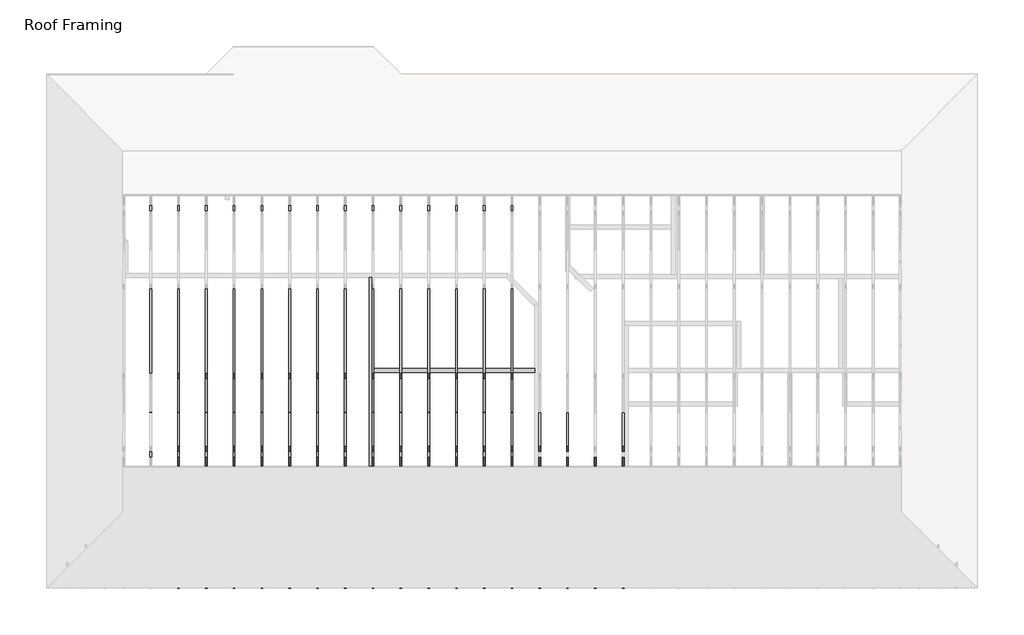
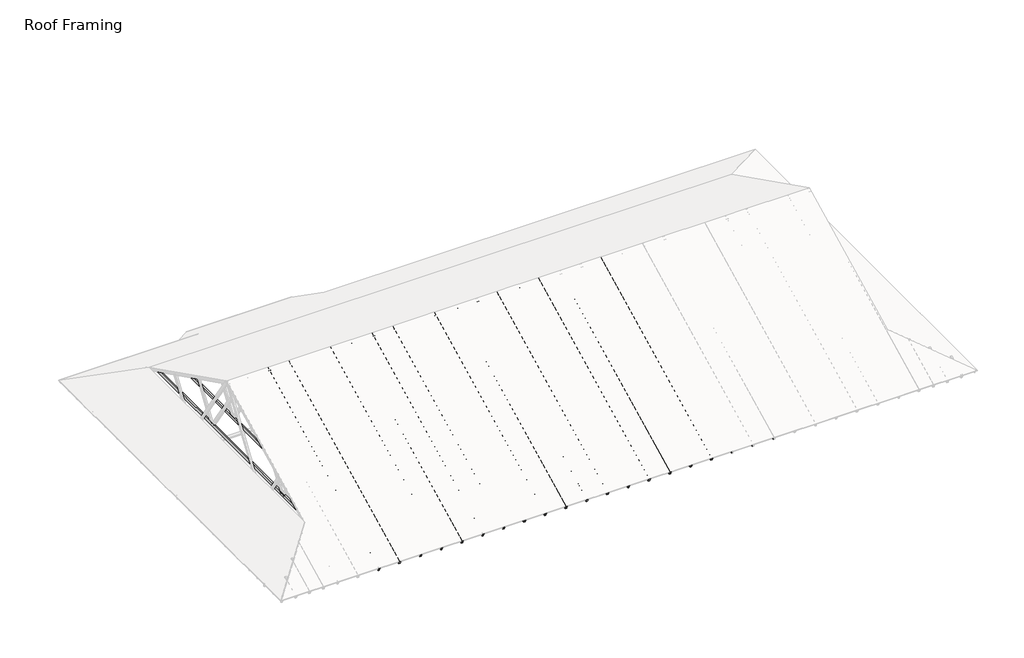
# One storey, part 2 of 7: 49 beams, 29 members.
"""IFC4 building model written with IfcOpenShell, lengths in millimetres."""

import ifcopenshell
import ifcopenshell.guid

model = None  # the IFC model being written
_history = None  # IfcOwnerHistory: only IFC2X3 demands one
_inside = {}  # id of a spatial element -> (the spatial element, [elements in it])
_under = {}  # id of a project, library or spatial element -> (it, [spatial elements below it])
_declared = {}  # id of a project -> (the project, [libraries it declares])
_typed = {}  # id of a type object -> (the type object, [elements of that type])
_made_of = {}  # id of a material, layer set ... -> (it, [elements and type objects made of it])


def new_model(schema):
    """Start an empty IFC model of exactly this schema.

    Asked for "IFC4X3", IfcOpenShell would pick the latest addendum, in which some entities
    have other attributes; the version numbers below select the first issue.
    IFC2X3 requires an IfcOwnerHistory on every rooted entity: one is made here for all.
    """
    global model, _history
    if schema == "IFC4X3":
        model = ifcopenshell.file(schema_version=(4, 3, 0, 0))
    else:
        model = ifcopenshell.file(schema=schema)
    _inside.clear()
    _under.clear()
    _declared.clear()
    _typed.clear()
    _made_of.clear()
    _history = None
    if model.schema == "IFC2X3":
        org = make("IfcOrganization", Name="unknown")
        user = make(
            "IfcPersonAndOrganization",
            ThePerson=make("IfcPerson", FamilyName="unknown"),
            TheOrganization=org,
        )
        app = make(
            "IfcApplication",
            ApplicationDeveloper=org,
            Version="unknown",
            ApplicationFullName="unknown",
            ApplicationIdentifier="unknown",
        )
        _history = make(
            "IfcOwnerHistory",
            OwningUser=user,
            OwningApplication=app,
            ChangeAction="ADDED",
            CreationDate=0,
        )
    return model


def make(cls, **values):
    """One entity of the class cls with the attributes given. An attribute that is None is left unset."""
    return model.create_entity(
        cls, **{name: value for name, value in values.items() if value is not None}
    )


def rooted(cls, **values):
    """An entity with a GlobalId (a new one), such as an element, a storey or a relation."""
    return make(cls, GlobalId=ifcopenshell.guid.new(), OwnerHistory=_history, **values)


def si_unit(unit_type, name, prefix=None):
    """IfcSIUnit, for example si_unit("LENGTHUNIT", "METRE", prefix="MILLI")."""
    return make("IfcSIUnit", UnitType=unit_type, Prefix=prefix, Name=name)


def assignment(units):
    """IfcUnitAssignment: the units of a project."""
    return None if units is None else make("IfcUnitAssignment", Units=units)


def point(xyz):
    """IfcCartesianPoint."""
    return None if xyz is None else make("IfcCartesianPoint", Coordinates=xyz)


def direction(xyz):
    """IfcDirection."""
    return None if xyz is None else make("IfcDirection", DirectionRatios=xyz)


def frame(location, z_axis=None, x_axis=None):
    """IfcAxis2Placement3D, a coordinate frame: its origin and axes. An axis left out is left unset."""
    return make(
        "IfcAxis2Placement3D",
        Location=point(location),
        Axis=direction(z_axis),
        RefDirection=direction(x_axis),
    )


def origin():
    """The frame at (0, 0, 0) with its axes left unset."""
    return frame((0.0, 0.0, 0.0))


def place(relative_to, where):
    """IfcLocalPlacement: puts the frame where relative to a parent placement (None: the world)."""
    return make(
        "IfcLocalPlacement", PlacementRelTo=relative_to, RelativePlacement=where
    )


def context(
    kind, dimensions, precision=None, world=None, true_north=None, identifier=None
):
    """IfcGeometricRepresentationContext, for example the 3D "Model" context."""
    return make(
        "IfcGeometricRepresentationContext",
        ContextIdentifier=identifier,
        ContextType=kind,
        CoordinateSpaceDimension=dimensions,
        Precision=precision,
        WorldCoordinateSystem=world,
        TrueNorth=true_north,
    )


def project(units=None, contexts=None):
    """IfcProject with its units and contexts."""
    return rooted(
        "IfcProject",
        Name="project",
        RepresentationContexts=contexts,
        UnitsInContext=assignment(units),
    )


def spatial(cls, under=None, at=None, **own):
    """A site, building, storey or space (cls), placed at a placement, below another one or the project."""
    s = rooted(cls, ObjectPlacement=at, **own)
    if under is not None:
        _under.setdefault(under.id(), (under, []))[1].append(s)
    return s


def polyline(points):
    """IfcPolyline through the points."""
    return make("IfcPolyline", Points=[point(p) for p in points])


def outline(outer, holes=None, kind="AREA"):
    """IfcArbitraryClosedProfileDef: a profile drawn as a closed curve; with holes, ...WithVoids."""
    if holes is None:
        return make("IfcArbitraryClosedProfileDef", ProfileType=kind, OuterCurve=outer)
    return make(
        "IfcArbitraryProfileDefWithVoids",
        ProfileType=kind,
        OuterCurve=outer,
        InnerCurves=holes,
    )


def extrude(swept, where, along, depth):
    """IfcExtrudedAreaSolid: the profile swept, set in the frame where, extruded along a direction by depth."""
    return make(
        "IfcExtrudedAreaSolid",
        SweptArea=swept,
        Position=where,
        ExtrudedDirection=direction(along),
        Depth=depth,
    )


def shape(context_of_items, identifier, shape_type, items):
    """IfcShapeRepresentation: the items that make up one representation, for example the "Body"."""
    return make(
        "IfcShapeRepresentation",
        ContextOfItems=context_of_items,
        RepresentationIdentifier=identifier,
        RepresentationType=shape_type,
        Items=items,
    )


def source(mapping_origin, context_of_items, identifier, shape_type, items):
    """IfcRepresentationMap: a shape defined once, which mapped items show again and again."""
    return make(
        "IfcRepresentationMap",
        MappingOrigin=mapping_origin,
        MappedRepresentation=shape(context_of_items, identifier, shape_type, items),
    )


def transform(
    local_origin,
    x_axis=None,
    y_axis=None,
    z_axis=None,
    scale=None,
    scale2=None,
    scale3=None,
    uniform=True,
):
    """IfcCartesianTransformationOperator3D, or its non-uniform kind. x_axis, y_axis, z_axis: its Axis1, 2, 3."""
    if uniform:
        return make(
            "IfcCartesianTransformationOperator3D",
            Axis1=direction(x_axis),
            Axis2=direction(y_axis),
            LocalOrigin=point(local_origin),
            Scale=scale,
            Axis3=direction(z_axis),
        )
    return make(
        "IfcCartesianTransformationOperator3DnonUniform",
        Axis1=direction(x_axis),
        Axis2=direction(y_axis),
        LocalOrigin=point(local_origin),
        Scale=scale,
        Axis3=direction(z_axis),
        Scale2=scale2,
        Scale3=scale3,
    )


def mapped(mapping_source, mapping_target):
    """IfcMappedItem: shows the shape of a source again, moved by a transform."""
    return make(
        "IfcMappedItem", MappingSource=mapping_source, MappingTarget=mapping_target
    )


def made_of(thing, what):
    """Note that an element or type object is made of a material, layer set ...; save() writes the relation."""
    if what is not None:
        _made_of.setdefault(what.id(), (what, []))[1].append(thing)
    return thing


def element(
    cls,
    number,
    at=None,
    inside=None,
    cuts=None,
    type_object=None,
    material=None,
    context=None,
    identifier="Body",
    shape_type=None,
    held_by="IfcProductDefinitionShape",
    body=None,
    shapes=None,
    **own,
):
    """One element of the class cls, such as IfcWall. Its Tag is "e" and its number.

    at: its placement. inside: the storey or other place that contains it. cuts: it is an
    opening in that element (IfcRelVoidsElement). A single representation is given by context,
    identifier, shape_type and body (its items); several are given by shapes. held_by: the class
    of the entity that holds the representations. save() writes the other relations.
    """
    e = rooted(cls, Tag="e%d" % number, ObjectPlacement=at, **own)
    if body is not None:
        shapes = [shape(context, identifier, shape_type, body)]
    if shapes is not None:
        e.Representation = make(held_by, Representations=shapes)
    if inside is not None:
        _inside.setdefault(inside.id(), (inside, []))[1].append(e)
    if cuts is not None:
        rooted(
            "IfcRelVoidsElement", RelatingBuildingElement=cuts, RelatedOpeningElement=e
        )
    if type_object is not None:
        _typed.setdefault(type_object.id(), (type_object, []))[1].append(e)
    return made_of(e, material)


def aggregate(whole, parts):
    """IfcRelAggregates: a whole, such as a stair, and the parts it consists of."""
    return rooted("IfcRelAggregates", RelatingObject=whole, RelatedObjects=parts)


def save(model, path):
    """Write the relations noted so far, then the file.

    IfcRelAggregates (storeys below a building ...), IfcRelContainedInSpatialStructure (elements
    in a storey), IfcRelDefinesByType, IfcRelAssociatesMaterial and IfcRelDeclares: one each for
    every whole, place, type object, material and project.
    """
    for whole, parts in _under.values():
        aggregate(whole, parts)
    for where, things in _inside.values():
        rooted(
            "IfcRelContainedInSpatialStructure",
            RelatedElements=things,
            RelatingStructure=where,
        )
    for kind, things in _typed.values():
        rooted("IfcRelDefinesByType", RelatedObjects=things, RelatingType=kind)
    for what, things in _made_of.values():
        rooted("IfcRelAssociatesMaterial", RelatedObjects=things, RelatingMaterial=what)
    for by, libraries in _declared.values():
        rooted("IfcRelDeclares", RelatingContext=by, RelatedDefinitions=libraries)
    model.write(path)


def dimension_lumber_f19b9f83(model_context):
    return source(origin(), model_context, "Body", "SweptSolid", [
        extrude(outline(polyline([(13763.625, -19.05), (-5743.575, -19.05), (-5743.575, 19.05), (13763.625, 19.05), (13763.625, -19.05)])), frame((0.0, 0.0, -44.45), z_axis=(0.0, 0.0, 1.0), x_axis=(1.0, 0.0, 0.0)), (0.0, 0.0, 1.0), 88.9),
    ])


def dimension_lumber_59ffca9e(model_context):
    return source(origin(), model_context, "Body", "SweptSolid", [
        extrude(outline(polyline([(1028.7, 44.45), (1028.7, -44.45), (-1028.7, -44.45), (-1028.7, 44.45), (1028.7, 44.45)])), frame((0.0, 0.0, -19.05), z_axis=(0.0, 0.0, 1.0), x_axis=(1.0, 0.0, 0.0)), (0.0, 0.0, 1.0), 38.1),
    ])


def dimension_lumber_a9f99430(model_context):
    return source(origin(), model_context, "Body", "SweptSolid", [
        extrude(outline(polyline([(1762.125, 44.45), (1762.125, -44.45), (-1778.0, -44.45), (-1778.0, 44.45), (1762.125, 44.45)])), frame((0.0, 0.0, -19.05), z_axis=(0.0, 0.0, 1.0), x_axis=(1.0, 0.0, 0.0)), (0.0, 0.0, 1.0), 38.1),
    ])


def dimension_lumber_f5869125(model_context):
    return source(origin(), model_context, "Body", "SweptSolid", [
        extrude(outline(polyline([(3033.7125, 44.45), (3033.7125, -44.45), (-3116.2625, -44.45), (-3116.2625, 44.45), (3033.7125, 44.45)])), frame((0.0, 0.0, -19.05), z_axis=(0.0, 0.0, 1.0), x_axis=(1.0, 0.0, 0.0)), (0.0, 0.0, 1.0), 38.1),
    ])


model = new_model("IFC4")

# Units and contexts
model_context = context("Model", 3, world=origin())
ifc_project = project(units=[si_unit("LENGTHUNIT", "METRE", prefix="MILLI")], contexts=[model_context])

# Site, building, storey
site = spatial("IfcSite", under=ifc_project)
building = spatial("IfcBuilding", under=site)
storey = spatial("IfcBuildingStorey", under=building, Name="Roof Framing", Elevation=2768.6)

# Beams
placement = place(None, origin())
dimension_lumber_shape = dimension_lumber_f19b9f83(model_context)
element("IfcBeam", 1, ObjectType="Dimension Lumber : Roof Lumbers", at=placement, inside=storey, context=model_context, shape_type="MappedRepresentation", body=[
    mapped(dimension_lumber_shape, transform((7511.6097749, -5882.9040947, 2609.05625), x_axis=(-1.0, 0.0, 0.0), y_axis=(0.0, -1.0, 0.0), z_axis=(0.0, 0.0, 1.0))),
])
dimension_lumber_2_shape = dimension_lumber_59ffca9e(model_context)
element("IfcBeam", 2, ObjectType="Dimension Lumber : Top Supporting Lumbers", at=placement, inside=storey, context=model_context, shape_type="MappedRepresentation", body=[
    mapped(dimension_lumber_2_shape, transform((5025.5847749, -4282.7040947, 2749.55), x_axis=(1.0, 0.0, 0.0), y_axis=(0.0, 1.0, 0.0), z_axis=(0.0, 0.0, 1.0))),
])
element("IfcBeam", 3, ObjectType="Dimension Lumber : Top Supporting Lumbers", at=placement, inside=storey, context=model_context, shape_type="MappedRepresentation", body=[
    mapped(dimension_lumber_2_shape, transform((5025.5847749, -4282.7040947, 2711.45), x_axis=(1.0, 0.0, 0.0), y_axis=(0.0, 1.0, 0.0), z_axis=(0.0, 0.0, 1.0))),
])
dimension_lumber_3_shape = dimension_lumber_a9f99430(model_context)
element("IfcBeam", 4, ObjectType="Dimension Lumber : Top Supporting Lumbers", at=placement, inside=storey, context=model_context, shape_type="MappedRepresentation", body=[
    mapped(dimension_lumber_3_shape, transform((2234.7597749, -1545.8540947, 2711.45), x_axis=(1.0, 0.0, 0.0), y_axis=(0.0, 1.0, 0.0), z_axis=(0.0, 0.0, 1.0))),
])
dimension_lumber_4_shape = dimension_lumber_f5869125(model_context)
element("IfcBeam", 5, ObjectType="Dimension Lumber : Top Supporting Lumbers", at=placement, inside=storey, context=model_context, shape_type="MappedRepresentation", body=[
    mapped(dimension_lumber_4_shape, transform((412.3097749, -2544.3915947, 2711.45), x_axis=(0.0, 1.0, 0.0), y_axis=(-1.0, 0.0, 0.0), z_axis=(0.0, 0.0, 1.0))),
])
element("IfcBeam", 6, ObjectType="Dimension Lumber : 2x4 Blocking", at=placement, inside=storey, context=model_context, shape_type="SweptSolid", body=[
    extrude(outline(polyline([(7787.8347749, -6282.9540947), (7749.7347749, -6282.9540947), (7749.7347749, -5901.9540947), (7787.8347749, -5901.9540947), (7787.8347749, -6282.9540947)])), frame((0.0, 0.0, 2564.60625), z_axis=(0.0, 0.0, 1.0), x_axis=(1.0, 0.0, 0.0)), (0.0, 0.0, 1.0), 88.9),
    extrude(outline(polyline([(-6083.9649001, 2653.50625), (-5901.9540947, 2653.50625), (-5901.9540947, 2564.60625), (-6261.7649001, 2564.60625), (-6083.9649001, 2653.50625)])), frame((7749.7347749, 0.0, 0.0), z_axis=(1.0, 0.0, 0.0), x_axis=(0.0, 1.0, 0.0)), (0.0, 0.0, 1.0), 38.1),
])
element("IfcBeam", 7, ObjectType="Dimension Lumber : 2x4 Blocking", at=placement, inside=storey, context=model_context, shape_type="SweptSolid", body=[
    extrude(outline(polyline([(7178.2347749, -6282.9540947), (7140.1347749, -6282.9540947), (7140.1347749, -5901.9540947), (7178.2347749, -5901.9540947), (7178.2347749, -6282.9540947)])), frame((0.0, 0.0, 2564.60625), z_axis=(0.0, 0.0, 1.0), x_axis=(1.0, 0.0, 0.0)), (0.0, 0.0, 1.0), 88.9),
    extrude(outline(polyline([(-6083.9649001, 2653.50625), (-5901.9540947, 2653.50625), (-5901.9540947, 2564.60625), (-6261.7649001, 2564.60625), (-6083.9649001, 2653.50625)])), frame((7140.1347749, 0.0, 0.0), z_axis=(1.0, 0.0, 0.0), x_axis=(0.0, 1.0, 0.0)), (0.0, 0.0, 1.0), 38.1),
])
element("IfcBeam", 8, ObjectType="Dimension Lumber : 2x4 Blocking", at=placement, inside=storey, context=model_context, shape_type="SweptSolid", body=[
    extrude(outline(polyline([(6568.6347749, -6282.9540947), (6530.5347749, -6282.9540947), (6530.5347749, -5901.9540947), (6568.6347749, -5901.9540947), (6568.6347749, -6282.9540947)])), frame((0.0, 0.0, 2564.60625), z_axis=(0.0, 0.0, 1.0), x_axis=(1.0, 0.0, 0.0)), (0.0, 0.0, 1.0), 88.9),
    extrude(outline(polyline([(-6083.9649001, 2653.50625), (-5901.9540947, 2653.50625), (-5901.9540947, 2564.60625), (-6261.7649001, 2564.60625), (-6083.9649001, 2653.50625)])), frame((6530.5347749, 0.0, 0.0), z_axis=(1.0, 0.0, 0.0), x_axis=(0.0, 1.0, 0.0)), (0.0, 0.0, 1.0), 38.1),
])
element("IfcBeam", 9, ObjectType="Dimension Lumber : 2x4 Blocking", at=placement, inside=storey, context=model_context, shape_type="SweptSolid", body=[
    extrude(outline(polyline([(5959.0347749, -6282.9540947), (5920.9347749, -6282.9540947), (5920.9347749, -5901.9540947), (5959.0347749, -5901.9540947), (5959.0347749, -6282.9540947)])), frame((0.0, 0.0, 2564.60625), z_axis=(0.0, 0.0, 1.0), x_axis=(1.0, 0.0, 0.0)), (0.0, 0.0, 1.0), 88.9),
    extrude(outline(polyline([(-6083.9649001, 2653.50625), (-5901.9540947, 2653.50625), (-5901.9540947, 2564.60625), (-6261.7649001, 2564.60625), (-6083.9649001, 2653.50625)])), frame((5920.9347749, 0.0, 0.0), z_axis=(1.0, 0.0, 0.0), x_axis=(0.0, 1.0, 0.0)), (0.0, 0.0, 1.0), 38.1),
])
element("IfcBeam", 10, ObjectType="Dimension Lumber : 2x4 Blocking", at=placement, inside=storey, context=model_context, shape_type="SweptSolid", body=[
    extrude(outline(polyline([(5349.4347749, -6282.9540947), (5311.3347749, -6282.9540947), (5311.3347749, -5901.9540947), (5349.4347749, -5901.9540947), (5349.4347749, -6282.9540947)])), frame((0.0, 0.0, 2564.60625), z_axis=(0.0, 0.0, 1.0), x_axis=(1.0, 0.0, 0.0)), (0.0, 0.0, 1.0), 88.9),
    extrude(outline(polyline([(-6083.9649001, 2653.50625), (-5901.9540947, 2653.50625), (-5901.9540947, 2564.60625), (-6261.7649001, 2564.60625), (-6083.9649001, 2653.50625)])), frame((5311.3347749, 0.0, 0.0), z_axis=(1.0, 0.0, 0.0), x_axis=(0.0, 1.0, 0.0)), (0.0, 0.0, 1.0), 38.1),
])
element("IfcBeam", 11, ObjectType="Dimension Lumber : 2x4 Blocking", at=placement, inside=storey, context=model_context, shape_type="SweptSolid", body=[
    extrude(outline(polyline([(4739.8347749, -6282.9540947), (4701.7347749, -6282.9540947), (4701.7347749, -5901.9540947), (4739.8347749, -5901.9540947), (4739.8347749, -6282.9540947)])), frame((0.0, 0.0, 2564.60625), z_axis=(0.0, 0.0, 1.0), x_axis=(1.0, 0.0, 0.0)), (0.0, 0.0, 1.0), 88.9),
    extrude(outline(polyline([(-6083.9649001, 2653.50625), (-5901.9540947, 2653.50625), (-5901.9540947, 2564.60625), (-6261.7649001, 2564.60625), (-6083.9649001, 2653.50625)])), frame((4701.7347749, 0.0, 0.0), z_axis=(1.0, 0.0, 0.0), x_axis=(0.0, 1.0, 0.0)), (0.0, 0.0, 1.0), 38.1),
])
element("IfcBeam", 12, ObjectType="Dimension Lumber : 2x4 Blocking", at=placement, inside=storey, context=model_context, shape_type="SweptSolid", body=[
    extrude(outline(polyline([(4130.2347749, -6282.9540947), (4092.1347749, -6282.9540947), (4092.1347749, -5901.9540947), (4130.2347749, -5901.9540947), (4130.2347749, -6282.9540947)])), frame((0.0, 0.0, 2564.60625), z_axis=(0.0, 0.0, 1.0), x_axis=(1.0, 0.0, 0.0)), (0.0, 0.0, 1.0), 88.9),
    extrude(outline(polyline([(-6083.9649001, 2653.50625), (-5901.9540947, 2653.50625), (-5901.9540947, 2564.60625), (-6261.7649001, 2564.60625), (-6083.9649001, 2653.50625)])), frame((4092.1347749, 0.0, 0.0), z_axis=(1.0, 0.0, 0.0), x_axis=(0.0, 1.0, 0.0)), (0.0, 0.0, 1.0), 38.1),
])
element("IfcBeam", 13, ObjectType="Dimension Lumber : 2x4 Blocking", at=placement, inside=storey, context=model_context, shape_type="SweptSolid", body=[
    extrude(outline(polyline([(3520.6347749, -6282.9540947), (3482.5347749, -6282.9540947), (3482.5347749, -5901.9540947), (3520.6347749, -5901.9540947), (3520.6347749, -6282.9540947)])), frame((0.0, 0.0, 2564.60625), z_axis=(0.0, 0.0, 1.0), x_axis=(1.0, 0.0, 0.0)), (0.0, 0.0, 1.0), 88.9),
    extrude(outline(polyline([(-6083.9649001, 2653.50625), (-5901.9540947, 2653.50625), (-5901.9540947, 2564.60625), (-6261.7649001, 2564.60625), (-6083.9649001, 2653.50625)])), frame((3482.5347749, 0.0, 0.0), z_axis=(1.0, 0.0, 0.0), x_axis=(0.0, 1.0, 0.0)), (0.0, 0.0, 1.0), 38.1),
])
element("IfcBeam", 14, ObjectType="Dimension Lumber : 2x4 Blocking", at=placement, inside=storey, context=model_context, shape_type="SweptSolid", body=[
    extrude(outline(polyline([(2911.0347749, -6282.9540947), (2872.9347749, -6282.9540947), (2872.9347749, -5901.9540947), (2911.0347749, -5901.9540947), (2911.0347749, -6282.9540947)])), frame((0.0, 0.0, 2564.60625), z_axis=(0.0, 0.0, 1.0), x_axis=(1.0, 0.0, 0.0)), (0.0, 0.0, 1.0), 88.9),
    extrude(outline(polyline([(-6083.9649001, 2653.50625), (-5901.9540947, 2653.50625), (-5901.9540947, 2564.60625), (-6261.7649001, 2564.60625), (-6083.9649001, 2653.50625)])), frame((2872.9347749, 0.0, 0.0), z_axis=(1.0, 0.0, 0.0), x_axis=(0.0, 1.0, 0.0)), (0.0, 0.0, 1.0), 38.1),
])
element("IfcBeam", 15, ObjectType="Dimension Lumber : 2x4 Blocking", at=placement, inside=storey, context=model_context, shape_type="SweptSolid", body=[
    extrude(outline(polyline([(2263.3347749, -5901.9540947), (2301.4347749, -5901.9540947), (2301.4347749, -6282.9540947), (2263.3347749, -6282.9540947), (2263.3347749, -5901.9540947)])), frame((0.0, 0.0, 2564.60625), z_axis=(0.0, 0.0, 1.0), x_axis=(1.0, 0.0, 0.0)), (0.0, 0.0, 1.0), 88.9),
    extrude(outline(polyline([(-5901.9540947, 2653.50625), (-5901.9540947, 2564.60625), (-6261.7649001, 2564.60625), (-6083.9649001, 2653.50625), (-5901.9540947, 2653.50625)])), frame((2263.3347749, 0.0, 0.0), z_axis=(1.0, 0.0, 0.0), x_axis=(0.0, 1.0, 0.0)), (0.0, 0.0, 1.0), 38.1),
])
element("IfcBeam", 16, ObjectType="Dimension Lumber : 2x4 Blocking", at=placement, inside=storey, context=model_context, shape_type="SweptSolid", body=[
    extrude(outline(polyline([(1653.7347749, -5901.9540947), (1691.8347749, -5901.9540947), (1691.8347749, -6282.9540947), (1653.7347749, -6282.9540947), (1653.7347749, -5901.9540947)])), frame((0.0, 0.0, 2564.60625), z_axis=(0.0, 0.0, 1.0), x_axis=(1.0, 0.0, 0.0)), (0.0, 0.0, 1.0), 88.9),
    extrude(outline(polyline([(-5901.9540947, 2653.50625), (-5901.9540947, 2564.60625), (-6261.7649001, 2564.60625), (-6083.9649001, 2653.50625), (-5901.9540947, 2653.50625)])), frame((1653.7347749, 0.0, 0.0), z_axis=(1.0, 0.0, 0.0), x_axis=(0.0, 1.0, 0.0)), (0.0, 0.0, 1.0), 38.1),
])
element("IfcBeam", 17, ObjectType="Dimension Lumber : 2x4 Blocking", at=placement, inside=storey, context=model_context, shape_type="SweptSolid", body=[
    extrude(outline(polyline([(1044.1347749, -5901.9540947), (1082.2347749, -5901.9540947), (1082.2347749, -6282.9540947), (1044.1347749, -6282.9540947), (1044.1347749, -5901.9540947)])), frame((0.0, 0.0, 2564.60625), z_axis=(0.0, 0.0, 1.0), x_axis=(1.0, 0.0, 0.0)), (0.0, 0.0, 1.0), 88.9),
    extrude(outline(polyline([(-5901.9540947, 2653.50625), (-5901.9540947, 2564.60625), (-6261.7649001, 2564.60625), (-6083.9649001, 2653.50625), (-5901.9540947, 2653.50625)])), frame((1044.1347749, 0.0, 0.0), z_axis=(1.0, 0.0, 0.0), x_axis=(0.0, 1.0, 0.0)), (0.0, 0.0, 1.0), 38.1),
])
element("IfcBeam", 18, ObjectType="Dimension Lumber : 2x4 Blocking", at=placement, inside=storey, context=model_context, shape_type="SweptSolid", body=[
    extrude(outline(polyline([(434.5347749, -5901.9540947), (472.6347749, -5901.9540947), (472.6347749, -6282.9540947), (434.5347749, -6282.9540947), (434.5347749, -5901.9540947)])), frame((0.0, 0.0, 2564.60625), z_axis=(0.0, 0.0, 1.0), x_axis=(1.0, 0.0, 0.0)), (0.0, 0.0, 1.0), 88.9),
    extrude(outline(polyline([(-5901.9540947, 2653.50625), (-5901.9540947, 2564.60625), (-6261.7649001, 2564.60625), (-6083.9649001, 2653.50625), (-5901.9540947, 2653.50625)])), frame((434.5347749, 0.0, 0.0), z_axis=(1.0, 0.0, 0.0), x_axis=(0.0, 1.0, 0.0)), (0.0, 0.0, 1.0), 38.1),
])
element("IfcBeam", 19, ObjectType="Dimension Lumber : 2x4 Truss", at=placement, inside=storey, context=model_context, shape_type="SweptSolid", body=[
    extrude(outline(polyline([(-682.2540947, 5453.7548743), (-682.2540947, 5354.3616527), (-6283.8372877, 2553.5700562), (-6323.5945763, 2633.0846335), (-682.2540947, 5453.7548743)])), frame((5920.9347749, 0.0, 0.0), z_axis=(1.0, 0.0, 0.0), x_axis=(0.0, 1.0, 0.0)), (0.0, 0.0, 1.0), 38.1),
])
element("IfcBeam", 20, ObjectType="Dimension Lumber : 2x4 Truss", at=placement, inside=storey, context=model_context, shape_type="SweptSolid", body=[
    extrude(outline(polyline([(-682.2540947, 5453.7548743), (-682.2540947, 5354.3616527), (-6283.8372877, 2553.5700562), (-6323.5945763, 2633.0846335), (-682.2540947, 5453.7548743)])), frame((5311.3347749, 0.0, 0.0), z_axis=(1.0, 0.0, 0.0), x_axis=(0.0, 1.0, 0.0)), (0.0, 0.0, 1.0), 38.1),
])
element("IfcBeam", 21, ObjectType="Dimension Lumber : 2x4 Truss", at=placement, inside=storey, context=model_context, shape_type="SweptSolid", body=[
    extrude(outline(polyline([(-682.2540947, 5453.7548743), (-682.2540947, 5354.3616527), (-6283.8372877, 2553.5700562), (-6323.5945763, 2633.0846335), (-682.2540947, 5453.7548743)])), frame((4701.7347749, 0.0, 0.0), z_axis=(1.0, 0.0, 0.0), x_axis=(0.0, 1.0, 0.0)), (0.0, 0.0, 1.0), 38.1),
])
element("IfcBeam", 22, ObjectType="Dimension Lumber : 2x4 Truss", at=placement, inside=storey, context=model_context, shape_type="SweptSolid", body=[
    extrude(outline(polyline([(-682.2540947, 5453.7548743), (-682.2540947, 5354.3616527), (-6283.8372877, 2553.5700562), (-6323.5945763, 2633.0846335), (-682.2540947, 5453.7548743)])), frame((4092.1347749, 0.0, 0.0), z_axis=(1.0, 0.0, 0.0), x_axis=(0.0, 1.0, 0.0)), (0.0, 0.0, 1.0), 38.1),
])
element("IfcBeam", 23, ObjectType="Dimension Lumber : 2x4 Truss", at=placement, inside=storey, context=model_context, shape_type="SweptSolid", body=[
    extrude(outline(polyline([(3520.6347749, -5876.623187), (3482.5347749, -5876.623187), (3482.5347749, 4488.2334053), (3520.6347749, 4488.2334053), (3520.6347749, -5876.623187)])), frame((0.0, 0.0, 2768.6), z_axis=(0.0, 0.0, 1.0), x_axis=(1.0, 0.0, 0.0)), (0.0, 0.0, 1.0), 88.9),
])
element("IfcBeam", 24, ObjectType="Dimension Lumber : 2x4 Truss", at=placement, inside=storey, context=model_context, shape_type="SweptSolid", body=[
    extrude(outline(polyline([(-682.2540947, 5453.7548743), (-682.2540947, 5354.3616527), (-6283.8372877, 2553.5700562), (-6323.5945763, 2633.0846335), (-682.2540947, 5453.7548743)])), frame((3482.5347749, 0.0, 0.0), z_axis=(1.0, 0.0, 0.0), x_axis=(0.0, 1.0, 0.0)), (0.0, 0.0, 1.0), 38.1),
])
element("IfcBeam", 25, ObjectType="Dimension Lumber : 2x4 Truss", at=placement, inside=storey, context=model_context, shape_type="SweptSolid", body=[
    extrude(outline(polyline([(2911.0347749, -5876.623187), (2872.9347749, -5876.623187), (2872.9347749, 4488.2334053), (2911.0347749, 4488.2334053), (2911.0347749, -5876.623187)])), frame((0.0, 0.0, 2768.6), z_axis=(0.0, 0.0, 1.0), x_axis=(1.0, 0.0, 0.0)), (0.0, 0.0, 1.0), 88.9),
])
element("IfcBeam", 26, ObjectType="Dimension Lumber : 2x4 Truss", at=placement, inside=storey, context=model_context, shape_type="SweptSolid", body=[
    extrude(outline(polyline([(-682.2540947, 5453.7548743), (-682.2540947, 5354.3616527), (-6283.8372877, 2553.5700562), (-6323.5945763, 2633.0846335), (-682.2540947, 5453.7548743)])), frame((2872.9347749, 0.0, 0.0), z_axis=(1.0, 0.0, 0.0), x_axis=(0.0, 1.0, 0.0)), (0.0, 0.0, 1.0), 38.1),
])
element("IfcBeam", 27, ObjectType="Dimension Lumber : 2x4 Truss", at=placement, inside=storey, context=model_context, shape_type="SweptSolid", body=[
    extrude(outline(polyline([(2301.4347749, -5876.623187), (2263.3347749, -5876.623187), (2263.3347749, 4488.2334053), (2301.4347749, 4488.2334053), (2301.4347749, -5876.623187)])), frame((0.0, 0.0, 2768.6), z_axis=(0.0, 0.0, 1.0), x_axis=(1.0, 0.0, 0.0)), (0.0, 0.0, 1.0), 88.9),
])
element("IfcBeam", 28, ObjectType="Dimension Lumber : 2x4 Truss", at=placement, inside=storey, context=model_context, shape_type="SweptSolid", body=[
    extrude(outline(polyline([(-682.2540947, 5453.7548743), (-682.2540947, 5354.3616527), (-6283.8372877, 2553.5700562), (-6323.5945763, 2633.0846335), (-682.2540947, 5453.7548743)])), frame((2263.3347749, 0.0, 0.0), z_axis=(1.0, 0.0, 0.0), x_axis=(0.0, 1.0, 0.0)), (0.0, 0.0, 1.0), 38.1),
])
element("IfcBeam", 29, ObjectType="Dimension Lumber : 2x4 Truss", at=placement, inside=storey, context=model_context, shape_type="SweptSolid", body=[
    extrude(outline(polyline([(1691.8347749, -5876.623187), (1653.7347749, -5876.623187), (1653.7347749, 4488.2334053), (1691.8347749, 4488.2334053), (1691.8347749, -5876.623187)])), frame((0.0, 0.0, 2768.6), z_axis=(0.0, 0.0, 1.0), x_axis=(1.0, 0.0, 0.0)), (0.0, 0.0, 1.0), 88.9),
])
element("IfcBeam", 30, ObjectType="Dimension Lumber : 2x4 Truss", at=placement, inside=storey, context=model_context, shape_type="SweptSolid", body=[
    extrude(outline(polyline([(-682.2540947, 5453.7548743), (-682.2540947, 5354.3616527), (-6283.8372877, 2553.5700562), (-6323.5945763, 2633.0846335), (-682.2540947, 5453.7548743)])), frame((1653.7347749, 0.0, 0.0), z_axis=(1.0, 0.0, 0.0), x_axis=(0.0, 1.0, 0.0)), (0.0, 0.0, 1.0), 38.1),
])
element("IfcBeam", 31, ObjectType="Dimension Lumber : 2x4 Truss", at=placement, inside=storey, context=model_context, shape_type="SweptSolid", body=[
    extrude(outline(polyline([(1082.2347749, -5876.623187), (1044.1347749, -5876.623187), (1044.1347749, 4488.2334053), (1082.2347749, 4488.2334053), (1082.2347749, -5876.623187)])), frame((0.0, 0.0, 2768.6), z_axis=(0.0, 0.0, 1.0), x_axis=(1.0, 0.0, 0.0)), (0.0, 0.0, 1.0), 88.9),
])
element("IfcBeam", 32, ObjectType="Dimension Lumber : 2x4 Truss", at=placement, inside=storey, context=model_context, shape_type="SweptSolid", body=[
    extrude(outline(polyline([(-682.2540947, 5453.7548743), (-682.2540947, 5354.3616527), (-6283.8372877, 2553.5700562), (-6323.5945763, 2633.0846335), (-682.2540947, 5453.7548743)])), frame((1044.1347749, 0.0, 0.0), z_axis=(1.0, 0.0, 0.0), x_axis=(0.0, 1.0, 0.0)), (0.0, 0.0, 1.0), 38.1),
])
element("IfcBeam", 33, ObjectType="Dimension Lumber : 2x4 Truss", at=placement, inside=storey, context=model_context, shape_type="SweptSolid", body=[
    extrude(outline(polyline([(472.6347749, -5876.623187), (434.5347749, -5876.623187), (434.5347749, 4488.2334053), (472.6347749, 4488.2334053), (472.6347749, -5876.623187)])), frame((0.0, 0.0, 2768.6), z_axis=(0.0, 0.0, 1.0), x_axis=(1.0, 0.0, 0.0)), (0.0, 0.0, 1.0), 88.9),
])
element("IfcBeam", 34, ObjectType="Dimension Lumber : 2x4 Truss", at=placement, inside=storey, context=model_context, shape_type="SweptSolid", body=[
    extrude(outline(polyline([(-682.2540947, 5453.7548743), (-682.2540947, 5354.3616527), (-6283.8372877, 2553.5700562), (-6323.5945763, 2633.0846335), (-682.2540947, 5453.7548743)])), frame((434.5347749, 0.0, 0.0), z_axis=(1.0, 0.0, 0.0), x_axis=(0.0, 1.0, 0.0)), (0.0, 0.0, 1.0), 38.1),
])
element("IfcBeam", 35, ObjectType="Dimension Lumber : 2x4 Truss", at=placement, inside=storey, context=model_context, shape_type="SweptSolid", body=[
    extrude(outline(polyline([(-136.9652251, -5876.623187), (-175.0652251, -5876.623187), (-175.0652251, 4488.2334053), (-136.9652251, 4488.2334053), (-136.9652251, -5876.623187)])), frame((0.0, 0.0, 2768.6), z_axis=(0.0, 0.0, 1.0), x_axis=(1.0, 0.0, 0.0)), (0.0, 0.0, 1.0), 88.9),
])
element("IfcBeam", 36, ObjectType="Dimension Lumber : 2x4 Truss", at=placement, inside=storey, context=model_context, shape_type="SweptSolid", body=[
    extrude(outline(polyline([(-682.2540947, 5453.7548743), (-682.2540947, 5354.3616527), (-6283.8372877, 2553.5700562), (-6323.5945763, 2633.0846335), (-682.2540947, 5453.7548743)])), frame((-175.0652251, 0.0, 0.0), z_axis=(1.0, 0.0, 0.0), x_axis=(0.0, 1.0, 0.0)), (0.0, 0.0, 1.0), 38.1),
])
element("IfcBeam", 37, ObjectType="Dimension Lumber : 2x4 Truss", at=placement, inside=storey, context=model_context, shape_type="SweptSolid", body=[
    extrude(outline(polyline([(-746.5652251, -5876.623187), (-784.6652251, -5876.623187), (-784.6652251, 4488.2334053), (-746.5652251, 4488.2334053), (-746.5652251, -5876.623187)])), frame((0.0, 0.0, 2768.6), z_axis=(0.0, 0.0, 1.0), x_axis=(1.0, 0.0, 0.0)), (0.0, 0.0, 1.0), 88.9),
])
element("IfcBeam", 38, ObjectType="Dimension Lumber : 2x4 Truss", at=placement, inside=storey, context=model_context, shape_type="SweptSolid", body=[
    extrude(outline(polyline([(-682.2540947, 5453.7548743), (-682.2540947, 5354.3616527), (-6283.8372877, 2553.5700562), (-6323.5945763, 2633.0846335), (-682.2540947, 5453.7548743)])), frame((-784.6652251, 0.0, 0.0), z_axis=(1.0, 0.0, 0.0), x_axis=(0.0, 1.0, 0.0)), (0.0, 0.0, 1.0), 38.1),
])
element("IfcBeam", 39, ObjectType="Dimension Lumber : 2x4 Truss", at=placement, inside=storey, context=model_context, shape_type="SweptSolid", body=[
    extrude(outline(polyline([(-1356.1652251, -5876.623187), (-1394.2652251, -5876.623187), (-1394.2652251, 4488.2334053), (-1356.1652251, 4488.2334053), (-1356.1652251, -5876.623187)])), frame((0.0, 0.0, 2768.6), z_axis=(0.0, 0.0, 1.0), x_axis=(1.0, 0.0, 0.0)), (0.0, 0.0, 1.0), 88.9),
])
element("IfcBeam", 40, ObjectType="Dimension Lumber : 2x4 Truss", at=placement, inside=storey, context=model_context, shape_type="SweptSolid", body=[
    extrude(outline(polyline([(-682.2540947, 5453.7548743), (-682.2540947, 5354.3616527), (-6283.8372877, 2553.5700562), (-6323.5945763, 2633.0846335), (-682.2540947, 5453.7548743)])), frame((-1394.2652251, 0.0, 0.0), z_axis=(1.0, 0.0, 0.0), x_axis=(0.0, 1.0, 0.0)), (0.0, 0.0, 1.0), 38.1),
])
element("IfcBeam", 41, ObjectType="Dimension Lumber : 2x4 Truss", at=placement, inside=storey, context=model_context, shape_type="SweptSolid", body=[
    extrude(outline(polyline([(-1965.7652251, -5876.623187), (-2003.8652251, -5876.623187), (-2003.8652251, 4488.2334053), (-1965.7652251, 4488.2334053), (-1965.7652251, -5876.623187)])), frame((0.0, 0.0, 2768.6), z_axis=(0.0, 0.0, 1.0), x_axis=(1.0, 0.0, 0.0)), (0.0, 0.0, 1.0), 88.9),
])
element("IfcBeam", 42, ObjectType="Dimension Lumber : 2x4 Truss", at=placement, inside=storey, context=model_context, shape_type="SweptSolid", body=[
    extrude(outline(polyline([(-682.2540947, 5453.7548743), (-682.2540947, 5354.3616527), (-6283.8372877, 2553.5700562), (-6323.5945763, 2633.0846335), (-682.2540947, 5453.7548743)])), frame((-2003.8652251, 0.0, 0.0), z_axis=(1.0, 0.0, 0.0), x_axis=(0.0, 1.0, 0.0)), (0.0, 0.0, 1.0), 38.1),
])
element("IfcBeam", 43, ObjectType="Dimension Lumber : 2x4 Truss", at=placement, inside=storey, context=model_context, shape_type="SweptSolid", body=[
    extrude(outline(polyline([(-2575.3652251, -5876.623187), (-2613.4652251, -5876.623187), (-2613.4652251, 4488.2334053), (-2575.3652251, 4488.2334053), (-2575.3652251, -5876.623187)])), frame((0.0, 0.0, 2768.6), z_axis=(0.0, 0.0, 1.0), x_axis=(1.0, 0.0, 0.0)), (0.0, 0.0, 1.0), 88.9),
])
element("IfcBeam", 44, ObjectType="Dimension Lumber : 2x4 Truss", at=placement, inside=storey, context=model_context, shape_type="SweptSolid", body=[
    extrude(outline(polyline([(-682.2540947, 5453.7548743), (-682.2540947, 5354.3616527), (-6283.8372877, 2553.5700562), (-6323.5945763, 2633.0846335), (-682.2540947, 5453.7548743)])), frame((-2613.4652251, 0.0, 0.0), z_axis=(1.0, 0.0, 0.0), x_axis=(0.0, 1.0, 0.0)), (0.0, 0.0, 1.0), 38.1),
])
element("IfcBeam", 45, ObjectType="Dimension Lumber : 2x4 Truss", at=placement, inside=storey, context=model_context, shape_type="SweptSolid", body=[
    extrude(outline(polyline([(-3184.9652251, -5876.623187), (-3223.0652251, -5876.623187), (-3223.0652251, 4488.2334053), (-3184.9652251, 4488.2334053), (-3184.9652251, -5876.623187)])), frame((0.0, 0.0, 2768.6), z_axis=(0.0, 0.0, 1.0), x_axis=(1.0, 0.0, 0.0)), (0.0, 0.0, 1.0), 88.9),
])
element("IfcBeam", 46, ObjectType="Dimension Lumber : 2x4 Truss", at=placement, inside=storey, context=model_context, shape_type="SweptSolid", body=[
    extrude(outline(polyline([(-682.2540947, 5453.7548743), (-682.2540947, 5354.3616527), (-6283.8372877, 2553.5700562), (-6323.5945763, 2633.0846335), (-682.2540947, 5453.7548743)])), frame((-3223.0652251, 0.0, 0.0), z_axis=(1.0, 0.0, 0.0), x_axis=(0.0, 1.0, 0.0)), (0.0, 0.0, 1.0), 38.1),
])
element("IfcBeam", 47, ObjectType="Dimension Lumber : 2x4 Truss", at=placement, inside=storey, context=model_context, shape_type="SweptSolid", body=[
    extrude(outline(polyline([(-3794.5652251, -5876.623187), (-3832.6652251, -5876.623187), (-3832.6652251, 4488.2334053), (-3794.5652251, 4488.2334053), (-3794.5652251, -5876.623187)])), frame((0.0, 0.0, 2768.6), z_axis=(0.0, 0.0, 1.0), x_axis=(1.0, 0.0, 0.0)), (0.0, 0.0, 1.0), 88.9),
])
element("IfcBeam", 48, ObjectType="Dimension Lumber : 2x4 Truss", at=placement, inside=storey, context=model_context, shape_type="SweptSolid", body=[
    extrude(outline(polyline([(-682.2540947, 5453.7548743), (-682.2540947, 5354.3616527), (-6283.8372877, 2553.5700562), (-6323.5945763, 2633.0846335), (-682.2540947, 5453.7548743)])), frame((-3832.6652251, 0.0, 0.0), z_axis=(1.0, 0.0, 0.0), x_axis=(0.0, 1.0, 0.0)), (0.0, 0.0, 1.0), 38.1),
])
element("IfcBeam", 49, ObjectType="Dimension Lumber : 2x4 Truss", at=placement, inside=storey, context=model_context, shape_type="SweptSolid", body=[
    extrude(outline(polyline([(-4404.1652251, -5876.623187), (-4442.2652251, -5876.623187), (-4442.2652251, 4488.2334053), (-4404.1652251, 4488.2334053), (-4404.1652251, -5876.623187)])), frame((0.0, 0.0, 2768.6), z_axis=(0.0, 0.0, 1.0), x_axis=(1.0, 0.0, 0.0)), (0.0, 0.0, 1.0), 88.9),
])

# Members
element("IfcMember", 50, ObjectType="Dimension Lumber : 2x4 Truss", at=placement, inside=storey, context=model_context, shape_type="SweptSolid", body=[
    extrude(outline(polyline([(44.4499999, 19.05), (44.4499999, -19.05), (-44.45, -19.05), (-44.45, 19.05), (44.4499999, 19.05)])), frame((5939.9847749, -2504.0569437, 2831.7897682), z_axis=(0.0, -0.5576002360134061, 0.8301096173384536), x_axis=(0.0, 0.8301096173384536, 0.5576002360134061)), (0.0, 0.0, 1.0), 1498.1463046),
])
element("IfcMember", 51, ObjectType="Dimension Lumber : 2x4 Truss", at=placement, inside=storey, context=model_context, shape_type="SweptSolid", body=[
    extrude(outline(polyline([(44.4499999, 19.05), (44.4499999, -19.05), (-44.45, -19.05), (-44.45, 19.05), (44.4499999, 19.05)])), frame((4720.7847749, -2504.0569437, 2831.7897682), z_axis=(0.0, -0.5576002360134061, 0.8301096173384536), x_axis=(0.0, 0.8301096173384536, 0.5576002360134061)), (0.0, 0.0, 1.0), 1498.1463046),
])
element("IfcMember", 52, ObjectType="Dimension Lumber : 2x4 Truss", at=placement, inside=storey, context=model_context, shape_type="SweptSolid", body=[
    extrude(outline(polyline([(44.4499999, 19.05), (44.4499999, -19.05), (-44.45, -19.05), (-44.45, 19.05), (44.4499999, 19.05)])), frame((4111.1847749, -2504.0569437, 2831.7897682), z_axis=(0.0, -0.5576002360134061, 0.8301096173384536), x_axis=(0.0, 0.8301096173384536, 0.5576002360134061)), (0.0, 0.0, 1.0), 1498.1463046),
])
element("IfcMember", 53, ObjectType="Dimension Lumber : 2x4 Truss", at=placement, inside=storey, context=model_context, shape_type="SweptSolid", body=[
    extrude(outline(polyline([(44.45, -19.05), (-44.45, -19.05), (-44.45, 19.05), (44.45, 19.05), (44.45, -19.05)])), frame((3501.5847749, -2430.2601988, 2831.7897682), z_axis=(0.0, 0.5576002360134061, 0.8301096173384536), x_axis=(0.0, -0.8301096173384536, 0.5576002360134061)), (0.0, 0.0, 1.0), 3068.6997979),
])
element("IfcMember", 54, ObjectType="Dimension Lumber : 2x4 Truss", at=placement, inside=storey, context=model_context, shape_type="SweptSolid", body=[
    extrude(outline(polyline([(44.4499999, 19.05), (44.4499999, -19.05), (-44.45, -19.05), (-44.45, 19.05), (44.4499999, 19.05)])), frame((3501.5847749, -2504.0569437, 2831.7897682), z_axis=(0.0, -0.5576002360134061, 0.8301096173384536), x_axis=(0.0, 0.8301096173384536, 0.5576002360134061)), (0.0, 0.0, 1.0), 1498.1463046),
])
element("IfcMember", 55, ObjectType="Dimension Lumber : 2x4 Truss", at=placement, inside=storey, context=model_context, shape_type="SweptSolid", body=[
    extrude(outline(polyline([(44.45, -19.05), (-44.45, -19.05), (-44.45, 19.05), (44.45, 19.05), (44.45, -19.05)])), frame((2891.9847749, -2430.2601988, 2831.7897682), z_axis=(0.0, 0.5576002360134061, 0.8301096173384536), x_axis=(0.0, -0.8301096173384536, 0.5576002360134061)), (0.0, 0.0, 1.0), 3068.6997979),
])
element("IfcMember", 56, ObjectType="Dimension Lumber : 2x4 Truss", at=placement, inside=storey, context=model_context, shape_type="SweptSolid", body=[
    extrude(outline(polyline([(44.4499999, 19.05), (44.4499999, -19.05), (-44.45, -19.05), (-44.45, 19.05), (44.4499999, 19.05)])), frame((2891.9847749, -2504.0569437, 2831.7897682), z_axis=(0.0, -0.5576002360134061, 0.8301096173384536), x_axis=(0.0, 0.8301096173384536, 0.5576002360134061)), (0.0, 0.0, 1.0), 1498.1463046),
])
element("IfcMember", 57, ObjectType="Dimension Lumber : 2x4 Truss", at=placement, inside=storey, context=model_context, shape_type="SweptSolid", body=[
    extrude(outline(polyline([(44.45, -19.05), (-44.45, -19.05), (-44.45, 19.05), (44.45, 19.05), (44.45, -19.05)])), frame((2282.3847749, -2430.2601988, 2831.7897682), z_axis=(0.0, 0.5576002360134061, 0.8301096173384536), x_axis=(0.0, -0.8301096173384536, 0.5576002360134061)), (0.0, 0.0, 1.0), 3068.6997979),
])
element("IfcMember", 58, ObjectType="Dimension Lumber : 2x4 Truss", at=placement, inside=storey, context=model_context, shape_type="SweptSolid", body=[
    extrude(outline(polyline([(44.4499999, 19.05), (44.4499999, -19.05), (-44.45, -19.05), (-44.45, 19.05), (44.4499999, 19.05)])), frame((2282.3847749, -2504.0569437, 2831.7897682), z_axis=(0.0, -0.5576002360134061, 0.8301096173384536), x_axis=(0.0, 0.8301096173384536, 0.5576002360134061)), (0.0, 0.0, 1.0), 1498.1463046),
])
element("IfcMember", 59, ObjectType="Dimension Lumber : 2x4 Truss", at=placement, inside=storey, context=model_context, shape_type="SweptSolid", body=[
    extrude(outline(polyline([(44.45, -19.05), (-44.45, -19.05), (-44.45, 19.05), (44.45, 19.05), (44.45, -19.05)])), frame((1672.7847749, -2430.2601988, 2831.7897682), z_axis=(0.0, 0.5576002360134061, 0.8301096173384536), x_axis=(0.0, -0.8301096173384536, 0.5576002360134061)), (0.0, 0.0, 1.0), 3068.6997979),
])
element("IfcMember", 60, ObjectType="Dimension Lumber : 2x4 Truss", at=placement, inside=storey, context=model_context, shape_type="SweptSolid", body=[
    extrude(outline(polyline([(44.4499999, 19.05), (44.4499999, -19.05), (-44.45, -19.05), (-44.45, 19.05), (44.4499999, 19.05)])), frame((1672.7847749, -2504.0569437, 2831.7897682), z_axis=(0.0, -0.5576002360134061, 0.8301096173384536), x_axis=(0.0, 0.8301096173384536, 0.5576002360134061)), (0.0, 0.0, 1.0), 1498.1463046),
])
element("IfcMember", 61, ObjectType="Dimension Lumber : 2x4 Truss", at=placement, inside=storey, context=model_context, shape_type="SweptSolid", body=[
    extrude(outline(polyline([(44.45, -19.05), (-44.45, -19.05), (-44.45, 19.05), (44.45, 19.05), (44.45, -19.05)])), frame((1063.1847749, -2430.2601988, 2831.7897682), z_axis=(0.0, 0.5576002360134061, 0.8301096173384536), x_axis=(0.0, -0.8301096173384536, 0.5576002360134061)), (0.0, 0.0, 1.0), 3068.6997979),
])
element("IfcMember", 62, ObjectType="Dimension Lumber : 2x4 Truss", at=placement, inside=storey, context=model_context, shape_type="SweptSolid", body=[
    extrude(outline(polyline([(44.4499999, 19.05), (44.4499999, -19.05), (-44.45, -19.05), (-44.45, 19.05), (44.4499999, 19.05)])), frame((1063.1847749, -2504.0569437, 2831.7897682), z_axis=(0.0, -0.5576002360134061, 0.8301096173384536), x_axis=(0.0, 0.8301096173384536, 0.5576002360134061)), (0.0, 0.0, 1.0), 1498.1463046),
])
element("IfcMember", 63, ObjectType="Dimension Lumber : 2x4 Truss", at=placement, inside=storey, context=model_context, shape_type="SweptSolid", body=[
    extrude(outline(polyline([(44.45, -19.05), (-44.45, -19.05), (-44.45, 19.05), (44.45, 19.05), (44.45, -19.05)])), frame((453.5847749, -2430.2601988, 2831.7897682), z_axis=(0.0, 0.5576002360134061, 0.8301096173384536), x_axis=(0.0, -0.8301096173384536, 0.5576002360134061)), (0.0, 0.0, 1.0), 3068.6997979),
])
element("IfcMember", 64, ObjectType="Dimension Lumber : 2x4 Truss", at=placement, inside=storey, context=model_context, shape_type="SweptSolid", body=[
    extrude(outline(polyline([(44.4499999, 19.05), (44.4499999, -19.05), (-44.45, -19.05), (-44.45, 19.05), (44.4499999, 19.05)])), frame((453.5847749, -2504.0569437, 2831.7897682), z_axis=(0.0, -0.5576002360134061, 0.8301096173384536), x_axis=(0.0, 0.8301096173384536, 0.5576002360134061)), (0.0, 0.0, 1.0), 1498.1463046),
])
element("IfcMember", 65, ObjectType="Dimension Lumber : 2x4 Truss", at=placement, inside=storey, context=model_context, shape_type="SweptSolid", body=[
    extrude(outline(polyline([(44.45, -19.05), (-44.45, -19.05), (-44.45, 19.05), (44.45, 19.05), (44.45, -19.05)])), frame((-156.0152251, -2430.2601988, 2831.7897682), z_axis=(0.0, 0.5576002360134061, 0.8301096173384536), x_axis=(0.0, -0.8301096173384536, 0.5576002360134061)), (0.0, 0.0, 1.0), 3068.6997979),
])
element("IfcMember", 66, ObjectType="Dimension Lumber : 2x4 Truss", at=placement, inside=storey, context=model_context, shape_type="SweptSolid", body=[
    extrude(outline(polyline([(44.4499999, 19.05), (44.4499999, -19.05), (-44.45, -19.05), (-44.45, 19.05), (44.4499999, 19.05)])), frame((-156.0152251, -2504.0569437, 2831.7897682), z_axis=(0.0, -0.5576002360134061, 0.8301096173384536), x_axis=(0.0, 0.8301096173384536, 0.5576002360134061)), (0.0, 0.0, 1.0), 1498.1463046),
])
element("IfcMember", 67, ObjectType="Dimension Lumber : 2x4 Truss", at=placement, inside=storey, context=model_context, shape_type="SweptSolid", body=[
    extrude(outline(polyline([(44.45, -19.05), (-44.45, -19.05), (-44.45, 19.05), (44.45, 19.05), (44.45, -19.05)])), frame((-765.6152251, -2430.2601988, 2831.7897682), z_axis=(0.0, 0.5576002360134061, 0.8301096173384536), x_axis=(0.0, -0.8301096173384536, 0.5576002360134061)), (0.0, 0.0, 1.0), 3068.6997979),
])
element("IfcMember", 68, ObjectType="Dimension Lumber : 2x4 Truss", at=placement, inside=storey, context=model_context, shape_type="SweptSolid", body=[
    extrude(outline(polyline([(44.4499999, 19.05), (44.4499999, -19.05), (-44.45, -19.05), (-44.45, 19.05), (44.4499999, 19.05)])), frame((-765.6152251, -2504.0569437, 2831.7897682), z_axis=(0.0, -0.5576002360134061, 0.8301096173384536), x_axis=(0.0, 0.8301096173384536, 0.5576002360134061)), (0.0, 0.0, 1.0), 1498.1463046),
])
element("IfcMember", 69, ObjectType="Dimension Lumber : 2x4 Truss", at=placement, inside=storey, context=model_context, shape_type="SweptSolid", body=[
    extrude(outline(polyline([(44.45, -19.05), (-44.45, -19.05), (-44.45, 19.05), (44.45, 19.05), (44.45, -19.05)])), frame((-1375.2152251, -2430.2601988, 2831.7897682), z_axis=(0.0, 0.5576002360134061, 0.8301096173384536), x_axis=(0.0, -0.8301096173384536, 0.5576002360134061)), (0.0, 0.0, 1.0), 3068.6997979),
])
element("IfcMember", 70, ObjectType="Dimension Lumber : 2x4 Truss", at=placement, inside=storey, context=model_context, shape_type="SweptSolid", body=[
    extrude(outline(polyline([(44.4499999, 19.05), (44.4499999, -19.05), (-44.45, -19.05), (-44.45, 19.05), (44.4499999, 19.05)])), frame((-1375.2152251, -2504.0569437, 2831.7897682), z_axis=(0.0, -0.5576002360134061, 0.8301096173384536), x_axis=(0.0, 0.8301096173384536, 0.5576002360134061)), (0.0, 0.0, 1.0), 1498.1463046),
])
element("IfcMember", 71, ObjectType="Dimension Lumber : 2x4 Truss", at=placement, inside=storey, context=model_context, shape_type="SweptSolid", body=[
    extrude(outline(polyline([(44.45, -19.05), (-44.45, -19.05), (-44.45, 19.05), (44.45, 19.05), (44.45, -19.05)])), frame((-1984.8152251, -2430.2601988, 2831.7897682), z_axis=(0.0, 0.5576002360134061, 0.8301096173384536), x_axis=(0.0, -0.8301096173384536, 0.5576002360134061)), (0.0, 0.0, 1.0), 3068.6997979),
])
element("IfcMember", 72, ObjectType="Dimension Lumber : 2x4 Truss", at=placement, inside=storey, context=model_context, shape_type="SweptSolid", body=[
    extrude(outline(polyline([(44.4499999, 19.05), (44.4499999, -19.05), (-44.45, -19.05), (-44.45, 19.05), (44.4499999, 19.05)])), frame((-1984.8152251, -2504.0569437, 2831.7897682), z_axis=(0.0, -0.5576002360134061, 0.8301096173384536), x_axis=(0.0, 0.8301096173384536, 0.5576002360134061)), (0.0, 0.0, 1.0), 1498.1463046),
])
element("IfcMember", 73, ObjectType="Dimension Lumber : 2x4 Truss", at=placement, inside=storey, context=model_context, shape_type="SweptSolid", body=[
    extrude(outline(polyline([(44.45, -19.05), (-44.45, -19.05), (-44.45, 19.05), (44.45, 19.05), (44.45, -19.05)])), frame((-2594.4152251, -2430.2601988, 2831.7897682), z_axis=(0.0, 0.5576002360134061, 0.8301096173384536), x_axis=(0.0, -0.8301096173384536, 0.5576002360134061)), (0.0, 0.0, 1.0), 3068.6997979),
])
element("IfcMember", 74, ObjectType="Dimension Lumber : 2x4 Truss", at=placement, inside=storey, context=model_context, shape_type="SweptSolid", body=[
    extrude(outline(polyline([(44.4499999, 19.05), (44.4499999, -19.05), (-44.45, -19.05), (-44.45, 19.05), (44.4499999, 19.05)])), frame((-2594.4152251, -2504.0569437, 2831.7897682), z_axis=(0.0, -0.5576002360134061, 0.8301096173384536), x_axis=(0.0, 0.8301096173384536, 0.5576002360134061)), (0.0, 0.0, 1.0), 1498.1463046),
])
element("IfcMember", 75, ObjectType="Dimension Lumber : 2x4 Truss", at=placement, inside=storey, context=model_context, shape_type="SweptSolid", body=[
    extrude(outline(polyline([(44.45, -19.05), (-44.45, -19.05), (-44.45, 19.05), (44.45, 19.05), (44.45, -19.05)])), frame((-3204.0152251, -2430.2601988, 2831.7897682), z_axis=(0.0, 0.5576002360134061, 0.8301096173384536), x_axis=(0.0, -0.8301096173384536, 0.5576002360134061)), (0.0, 0.0, 1.0), 3068.6997979),
])
element("IfcMember", 76, ObjectType="Dimension Lumber : 2x4 Truss", at=placement, inside=storey, context=model_context, shape_type="SweptSolid", body=[
    extrude(outline(polyline([(44.4499999, 19.05), (44.4499999, -19.05), (-44.45, -19.05), (-44.45, 19.05), (44.4499999, 19.05)])), frame((-3204.0152251, -2504.0569437, 2831.7897682), z_axis=(0.0, -0.5576002360134061, 0.8301096173384536), x_axis=(0.0, 0.8301096173384536, 0.5576002360134061)), (0.0, 0.0, 1.0), 1498.1463046),
])
element("IfcMember", 77, ObjectType="Dimension Lumber : 2x4 Truss", at=placement, inside=storey, context=model_context, shape_type="SweptSolid", body=[
    extrude(outline(polyline([(44.45, -19.05), (-44.45, -19.05), (-44.45, 19.05), (44.45, 19.05), (44.45, -19.05)])), frame((-3813.6152251, -2430.2601988, 2831.7897682), z_axis=(0.0, 0.5576002360134061, 0.8301096173384536), x_axis=(0.0, -0.8301096173384536, 0.5576002360134061)), (0.0, 0.0, 1.0), 3068.6997979),
])
element("IfcMember", 78, ObjectType="Dimension Lumber : 2x4 Truss", at=placement, inside=storey, context=model_context, shape_type="SweptSolid", body=[
    extrude(outline(polyline([(44.4499999, 19.05), (44.4499999, -19.05), (-44.45, -19.05), (-44.45, 19.05), (44.4499999, 19.05)])), frame((-3813.6152251, -2504.0569437, 2831.7897682), z_axis=(0.0, -0.5576002360134061, 0.8301096173384536), x_axis=(0.0, 0.8301096173384536, 0.5576002360134061)), (0.0, 0.0, 1.0), 1498.1463046),
])

save(model, "model.ifc")

# Revit data of these elements
# Type "Dimension Lumber : Roof Lumbers"
#   Assembly Code = "B10"
#   A = 0.0364583 SF
#   Length [instance default] = 5' - 0"
#   b = 0' - 1 1/2"
#   d = 0' - 3 1/2"
#   Structural Material [instance default] = Softwood, Lumber
# Type "Dimension Lumber : Top Supporting Lumbers"
#   Assembly Code = "B10"
#   A = 0.0364583 SF
#   Length [instance default] = 5' - 0"
#   b = 0' - 3 1/2"
#   d = 0' - 1 1/2"
#   Structural Material [instance default] = Softwood, Lumber
# Type "Dimension Lumber : 2x4 Blocking"
#   Assembly Code = "B10"
#   Cost = 0
#   A = 0.0364583 SF
#   Length [instance default] = 5' - 0"
#   b = 0' - 1 1/2"
#   d = 0' - 3 1/2"
#   Structural Material [instance default] = Softwood, Lumber
# Type "Dimension Lumber : 2x4 Truss"
#   Assembly Code = "B10"
#   Cost = 750
#   A = 0.0364583 SF
#   Length [instance default] = 5' - 0"
#   b = 0' - 1 1/2"
#   d = 0' - 3 1/2"
#   Structural Material [instance default] = Softwood, Lumber
# Element 1 (IfcBeam, "Dimension Lumber : Roof Lumbers")
#   Structural Material = Douglas Fir #2
#   Phase Created = New Construction
#   Materials on its faces: "Douglas Fir #2"
# Elements 2, 3, 4, 5 (IfcBeam, "Dimension Lumber : Top Supporting Lumbers")
#   Structural Material = Douglas Fir #2
#   Phase Created = New Construction
#   Materials on its faces: "Douglas Fir #2"
# Elements 6, 7, 8, 9, 10, 11, 12, 13, 14, 15, 16, 17, 18 (IfcBeam, "Dimension Lumber : 2x4 Blocking")
#   Comments = ""
#   Structural Material = Douglas Fir #2
#   Phase Created = New Construction
#   Materials on its faces: "Douglas Fir #2"
# Elements 19, 20, 21, 22, 24, 26, 28, 30, 32, 34, 36, 38, 40, 42, 44, 46, 48 (IfcBeam, "Dimension Lumber : 2x4 Truss")
#   Structural Material = Douglas Fir #2
#   Phase Created = New Construction
#   Materials on its faces: "Douglas Fir #2"
# Elements 23, 25, 27, 29, 31, 33, 35, 37, 39, 41, 43, 45, 47, 49 (IfcBeam, "Dimension Lumber : 2x4 Truss")
#   Comments = ""
#   Structural Material = Douglas Fir #2
#   Phase Created = New Construction
#   Materials on its faces: "Douglas Fir #2"
# Elements 50, 51, 52, 53, 54, 55, 56, 57, 58, 59, 60, 61, 62, 63, 64, 65, 66, 67, 68, 69, 70, 71, 72, 73, 74, 75, 76, 77, 78 (IfcMember, "Dimension Lumber : 2x4 Truss")
#   Comments = ""
#   Structural Material = Douglas Fir #2
#   Phase Created = New Construction
#   Materials on its faces: "Douglas Fir #2"
# Materials
#   "Softwood, Lumber": class "Wood", colour RGB 223 192 134, transparency 0, Description = "Pinus Echinata", Cost = 0
#   "Douglas Fir #2": class "Wood", colour RGB 223 192 134, transparency 0, Description = "Pinus Echinata", Cost = 0
